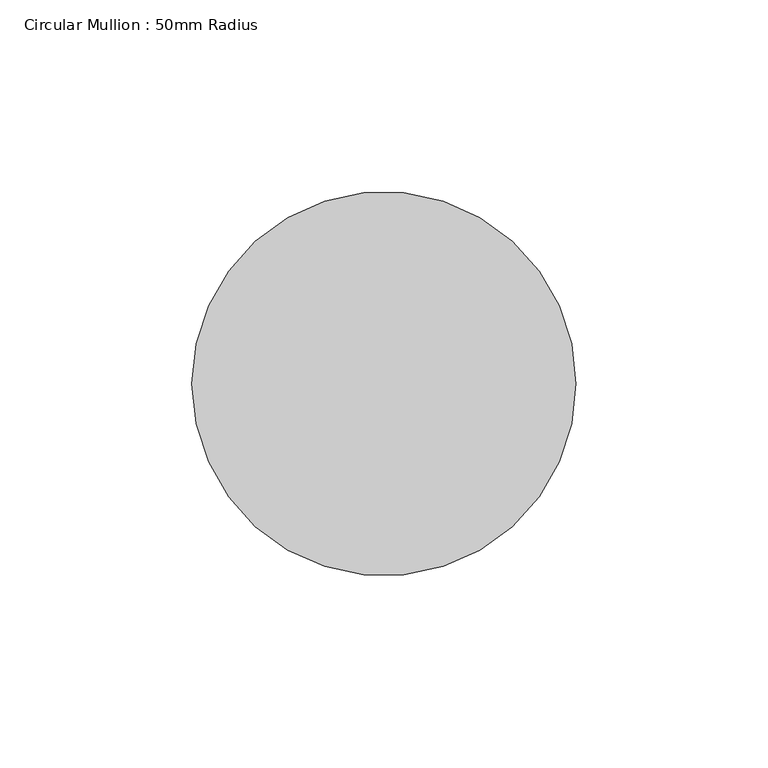
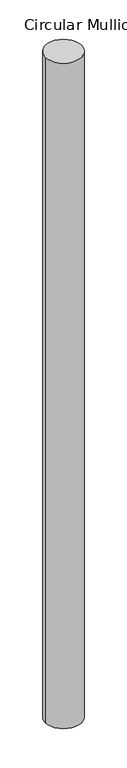
"""IFC4 building model written with IfcOpenShell, lengths in millimetres: member geometry, Circular Mullion : 50mm Radius."""

from ifc_helpers import new_model, si_unit, point, frame, frame_2d, origin, place, context, project, spatial, circle_curve, trimmed, segment, composite_curve, outline, extrude, source, transform, mapped, element, save


def circular_mullion_50mm_radius_062e0494(model_context):
    return source(origin(), model_context, "Body", "SweptSolid", [
        extrude(outline(composite_curve([segment(trimmed(circle_curve(frame_2d((-50.0, 0.0)), 50.0), [point((0.0, 0.0))], [point((-100.0, 0.0))], False, "CARTESIAN"), True, "CONTINUOUS"), segment(trimmed(circle_curve(frame_2d((-50.0, 0.0)), 50.0), [point((-100.0, 0.0))], [point((0.0, 0.0))], False, "CARTESIAN"), True, "CONTINUOUS")], self_intersect=False)), frame((0.0, 0.0, -1944.0907297), z_axis=(0.0, 0.0, 1.0), x_axis=(1.0, 0.0, 0.0)), (0.0, 0.0, 1.0), 1944.0907297),
    ])


if __name__ == "__main__":
    model = new_model("IFC4")
    model_context = context("Model", 3, world=origin())
    ifc_project = project(units=[si_unit("LENGTHUNIT", "METRE", prefix="MILLI")], contexts=[model_context])
    site = spatial("IfcSite", under=ifc_project)
    building = spatial("IfcBuilding", under=site)
    placement = place(None, origin())
    circular_mullion_50mm_radius_shape = circular_mullion_50mm_radius_062e0494(model_context)
    element("IfcMember", 1, ObjectType="Circular Mullion : 50mm Radius", at=placement, inside=building, context=model_context, shape_type="MappedRepresentation", body=[
        mapped(circular_mullion_50mm_radius_shape, transform((0.0, 0.0, 0.0), x_axis=(1.0, 0.0, 0.0), y_axis=(0.0, 1.0, 0.0), z_axis=(0.0, 0.0, 1.0))),
    ])
    save(model, "model.ifc")

# Revit data of these elements
# Type "Circular Mullion : 50mm Radius"
#   built-in parameter 1007350 = 0.164042 (stored number, unit not read)
# Element 1 (IfcMember, "Circular Mullion : 50mm Radius")
#   Materials on its faces: "Aluminium"
# Materials
#   "Aluminium": class "Metal", colour RGB 247 247 247, transparency 0, Description = "Aluminium 6061", Cost = 0
